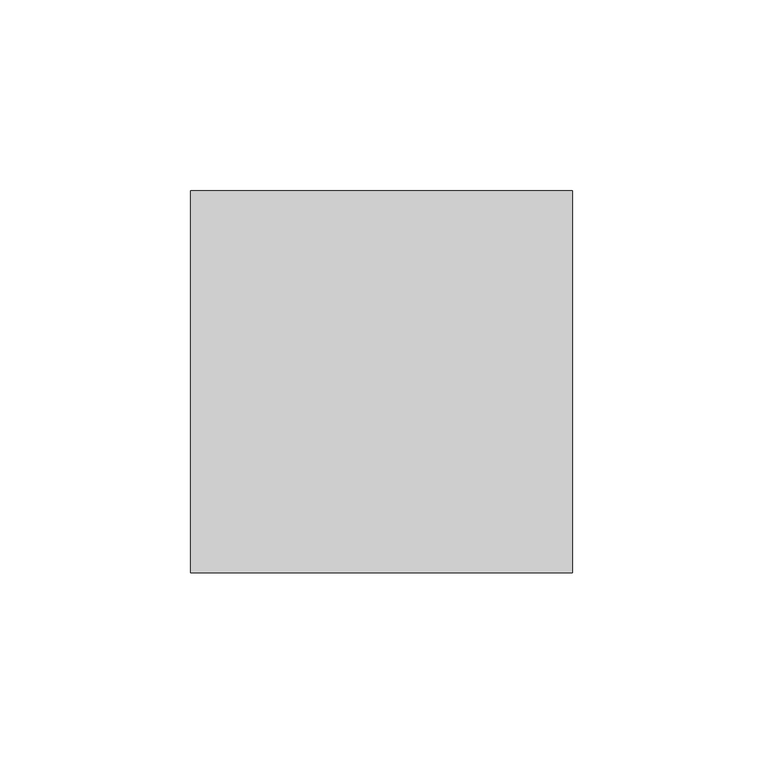
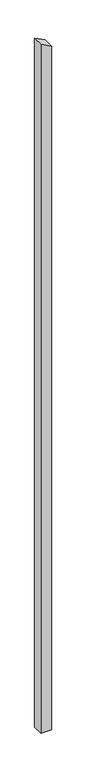
"""IFC4 building model written with IfcOpenShell, lengths in millimetres: column geometry, Holzstütze 159056 : Holzstütze 159056."""

import ifcopenshell
import ifcopenshell.guid

model = None  # the IFC model being written
_history = None  # IfcOwnerHistory: only IFC2X3 demands one
_inside = {}  # id of a spatial element -> (the spatial element, [elements in it])
_under = {}  # id of a project, library or spatial element -> (it, [spatial elements below it])
_declared = {}  # id of a project -> (the project, [libraries it declares])
_typed = {}  # id of a type object -> (the type object, [elements of that type])
_made_of = {}  # id of a material, layer set ... -> (it, [elements and type objects made of it])


def new_model(schema):
    """Start an empty IFC model of exactly this schema.

    Asked for "IFC4X3", IfcOpenShell would pick the latest addendum, in which some entities
    have other attributes; the version numbers below select the first issue.
    IFC2X3 requires an IfcOwnerHistory on every rooted entity: one is made here for all.
    """
    global model, _history
    if schema == "IFC4X3":
        model = ifcopenshell.file(schema_version=(4, 3, 0, 0))
    else:
        model = ifcopenshell.file(schema=schema)
    _inside.clear()
    _under.clear()
    _declared.clear()
    _typed.clear()
    _made_of.clear()
    _history = None
    if model.schema == "IFC2X3":
        org = make("IfcOrganization", Name="unknown")
        user = make(
            "IfcPersonAndOrganization",
            ThePerson=make("IfcPerson", FamilyName="unknown"),
            TheOrganization=org,
        )
        app = make(
            "IfcApplication",
            ApplicationDeveloper=org,
            Version="unknown",
            ApplicationFullName="unknown",
            ApplicationIdentifier="unknown",
        )
        _history = make(
            "IfcOwnerHistory",
            OwningUser=user,
            OwningApplication=app,
            ChangeAction="ADDED",
            CreationDate=0,
        )
    return model


def make(cls, **values):
    """One entity of the class cls with the attributes given. An attribute that is None is left unset."""
    return model.create_entity(
        cls, **{name: value for name, value in values.items() if value is not None}
    )


def rooted(cls, **values):
    """An entity with a GlobalId (a new one), such as an element, a storey or a relation."""
    return make(cls, GlobalId=ifcopenshell.guid.new(), OwnerHistory=_history, **values)


def si_unit(unit_type, name, prefix=None):
    """IfcSIUnit, for example si_unit("LENGTHUNIT", "METRE", prefix="MILLI")."""
    return make("IfcSIUnit", UnitType=unit_type, Prefix=prefix, Name=name)


def assignment(units):
    """IfcUnitAssignment: the units of a project."""
    return None if units is None else make("IfcUnitAssignment", Units=units)


def point(xyz):
    """IfcCartesianPoint."""
    return None if xyz is None else make("IfcCartesianPoint", Coordinates=xyz)


def direction(xyz):
    """IfcDirection."""
    return None if xyz is None else make("IfcDirection", DirectionRatios=xyz)


def frame(location, z_axis=None, x_axis=None):
    """IfcAxis2Placement3D, a coordinate frame: its origin and axes. An axis left out is left unset."""
    return make(
        "IfcAxis2Placement3D",
        Location=point(location),
        Axis=direction(z_axis),
        RefDirection=direction(x_axis),
    )


def origin():
    """The frame at (0, 0, 0) with its axes left unset."""
    return frame((0.0, 0.0, 0.0))


def place(relative_to, where):
    """IfcLocalPlacement: puts the frame where relative to a parent placement (None: the world)."""
    return make(
        "IfcLocalPlacement", PlacementRelTo=relative_to, RelativePlacement=where
    )


def context(
    kind, dimensions, precision=None, world=None, true_north=None, identifier=None
):
    """IfcGeometricRepresentationContext, for example the 3D "Model" context."""
    return make(
        "IfcGeometricRepresentationContext",
        ContextIdentifier=identifier,
        ContextType=kind,
        CoordinateSpaceDimension=dimensions,
        Precision=precision,
        WorldCoordinateSystem=world,
        TrueNorth=true_north,
    )


def project(units=None, contexts=None):
    """IfcProject with its units and contexts."""
    return rooted(
        "IfcProject",
        Name="project",
        RepresentationContexts=contexts,
        UnitsInContext=assignment(units),
    )


def spatial(cls, under=None, at=None, **own):
    """A site, building, storey or space (cls), placed at a placement, below another one or the project."""
    s = rooted(cls, ObjectPlacement=at, **own)
    if under is not None:
        _under.setdefault(under.id(), (under, []))[1].append(s)
    return s


def polyline(points):
    """IfcPolyline through the points."""
    return make("IfcPolyline", Points=[point(p) for p in points])


def outline(outer, holes=None, kind="AREA"):
    """IfcArbitraryClosedProfileDef: a profile drawn as a closed curve; with holes, ...WithVoids."""
    if holes is None:
        return make("IfcArbitraryClosedProfileDef", ProfileType=kind, OuterCurve=outer)
    return make(
        "IfcArbitraryProfileDefWithVoids",
        ProfileType=kind,
        OuterCurve=outer,
        InnerCurves=holes,
    )


def extrude(swept, where, along, depth):
    """IfcExtrudedAreaSolid: the profile swept, set in the frame where, extruded along a direction by depth."""
    return make(
        "IfcExtrudedAreaSolid",
        SweptArea=swept,
        Position=where,
        ExtrudedDirection=direction(along),
        Depth=depth,
    )


def shape(context_of_items, identifier, shape_type, items):
    """IfcShapeRepresentation: the items that make up one representation, for example the "Body"."""
    return make(
        "IfcShapeRepresentation",
        ContextOfItems=context_of_items,
        RepresentationIdentifier=identifier,
        RepresentationType=shape_type,
        Items=items,
    )


def source(mapping_origin, context_of_items, identifier, shape_type, items):
    """IfcRepresentationMap: a shape defined once, which mapped items show again and again."""
    return make(
        "IfcRepresentationMap",
        MappingOrigin=mapping_origin,
        MappedRepresentation=shape(context_of_items, identifier, shape_type, items),
    )


def transform(
    local_origin,
    x_axis=None,
    y_axis=None,
    z_axis=None,
    scale=None,
    scale2=None,
    scale3=None,
    uniform=True,
):
    """IfcCartesianTransformationOperator3D, or its non-uniform kind. x_axis, y_axis, z_axis: its Axis1, 2, 3."""
    if uniform:
        return make(
            "IfcCartesianTransformationOperator3D",
            Axis1=direction(x_axis),
            Axis2=direction(y_axis),
            LocalOrigin=point(local_origin),
            Scale=scale,
            Axis3=direction(z_axis),
        )
    return make(
        "IfcCartesianTransformationOperator3DnonUniform",
        Axis1=direction(x_axis),
        Axis2=direction(y_axis),
        LocalOrigin=point(local_origin),
        Scale=scale,
        Axis3=direction(z_axis),
        Scale2=scale2,
        Scale3=scale3,
    )


def mapped(mapping_source, mapping_target):
    """IfcMappedItem: shows the shape of a source again, moved by a transform."""
    return make(
        "IfcMappedItem", MappingSource=mapping_source, MappingTarget=mapping_target
    )


def made_of(thing, what):
    """Note that an element or type object is made of a material, layer set ...; save() writes the relation."""
    if what is not None:
        _made_of.setdefault(what.id(), (what, []))[1].append(thing)
    return thing


def element(
    cls,
    number,
    at=None,
    inside=None,
    cuts=None,
    type_object=None,
    material=None,
    context=None,
    identifier="Body",
    shape_type=None,
    held_by="IfcProductDefinitionShape",
    body=None,
    shapes=None,
    **own,
):
    """One element of the class cls, such as IfcWall. Its Tag is "e" and its number.

    at: its placement. inside: the storey or other place that contains it. cuts: it is an
    opening in that element (IfcRelVoidsElement). A single representation is given by context,
    identifier, shape_type and body (its items); several are given by shapes. held_by: the class
    of the entity that holds the representations. save() writes the other relations.
    """
    e = rooted(cls, Tag="e%d" % number, ObjectPlacement=at, **own)
    if body is not None:
        shapes = [shape(context, identifier, shape_type, body)]
    if shapes is not None:
        e.Representation = make(held_by, Representations=shapes)
    if inside is not None:
        _inside.setdefault(inside.id(), (inside, []))[1].append(e)
    if cuts is not None:
        rooted(
            "IfcRelVoidsElement", RelatingBuildingElement=cuts, RelatedOpeningElement=e
        )
    if type_object is not None:
        _typed.setdefault(type_object.id(), (type_object, []))[1].append(e)
    return made_of(e, material)


def aggregate(whole, parts):
    """IfcRelAggregates: a whole, such as a stair, and the parts it consists of."""
    return rooted("IfcRelAggregates", RelatingObject=whole, RelatedObjects=parts)


def save(model, path):
    """Write the relations noted so far, then the file.

    IfcRelAggregates (storeys below a building ...), IfcRelContainedInSpatialStructure (elements
    in a storey), IfcRelDefinesByType, IfcRelAssociatesMaterial and IfcRelDeclares: one each for
    every whole, place, type object, material and project.
    """
    for whole, parts in _under.values():
        aggregate(whole, parts)
    for where, things in _inside.values():
        rooted(
            "IfcRelContainedInSpatialStructure",
            RelatedElements=things,
            RelatingStructure=where,
        )
    for kind, things in _typed.values():
        rooted("IfcRelDefinesByType", RelatedObjects=things, RelatingType=kind)
    for what, things in _made_of.values():
        rooted("IfcRelAssociatesMaterial", RelatedObjects=things, RelatingMaterial=what)
    for by, libraries in _declared.values():
        rooted("IfcRelDeclares", RelatingContext=by, RelatedDefinitions=libraries)
    model.write(path)


def column_ed14f447(model_context):
    return source(origin(), model_context, "Body", "SweptSolid", [
        extrude(outline(polyline([(-500.0, 174197.7593015), (-500.0, 174297.7593015), (6345.7118258, 174297.7593015), (6396.6643707, 174197.7593015), (-500.0, 174197.7593015)])), frame((0.0, 29551.5369795, 0.0), z_axis=(0.0, 1.0, 0.0), x_axis=(0.0, 0.0, 1.0)), (0.0, 0.0, 1.0), 100.0),
    ])


if __name__ == "__main__":
    model = new_model("IFC4")
    model_context = context("Model", 3, world=origin())
    ifc_project = project(units=[si_unit("LENGTHUNIT", "METRE", prefix="MILLI")], contexts=[model_context])
    site = spatial("IfcSite", under=ifc_project)
    building = spatial("IfcBuilding", under=site)
    placement = place(None, origin())
    column_shape = column_ed14f447(model_context)
    element("IfcColumn", 1, ObjectType="Holzstütze 159056 : Holzstütze 159056", at=placement, inside=building, context=model_context, shape_type="MappedRepresentation", body=[
        mapped(column_shape, transform((0.0, 0.0, 0.0), x_axis=(1.0, 0.0, 0.0), y_axis=(0.0, 1.0, 0.0), z_axis=(0.0, 0.0, 1.0))),
    ])
    save(model, "model.ifc")

# Revit data of these elements
# Type "Holzstütze 159056 : Holzstütze 159056"
#   Abrechnungsart = "m"
#   Allright_Bauteil_ID = "0152St 0000143490"
#   Bezeichnung = "Holzstütze"
#   Codetext = "ST-HOLZ\\"
#   Gewerk = "Zimmer- und Holzbauarbeiten"
#   Material = "Holz"
#   Objektname = "Stütze"
#   NameOverride = "Holzstütze"
#   Reference = "Holzstütze"
#   Status = "NEW"
#   ThermalTransmittance = 0.0000 BTU/(h·ft²·°F)
#   Roll = 0.00°
#   Slope = 0.00°
#   2D Interaktion = yes
#   IsExternal = yes
#   LoadBearing = yes
# Element 1 (IfcColumn, "Holzstütze 159056 : Holzstütze 159056")
#   Materials on its faces: "holzschalung"
# Materials
#   "holzschalung": class "Unassigned", colour RGB 128 128 128, transparency 0
